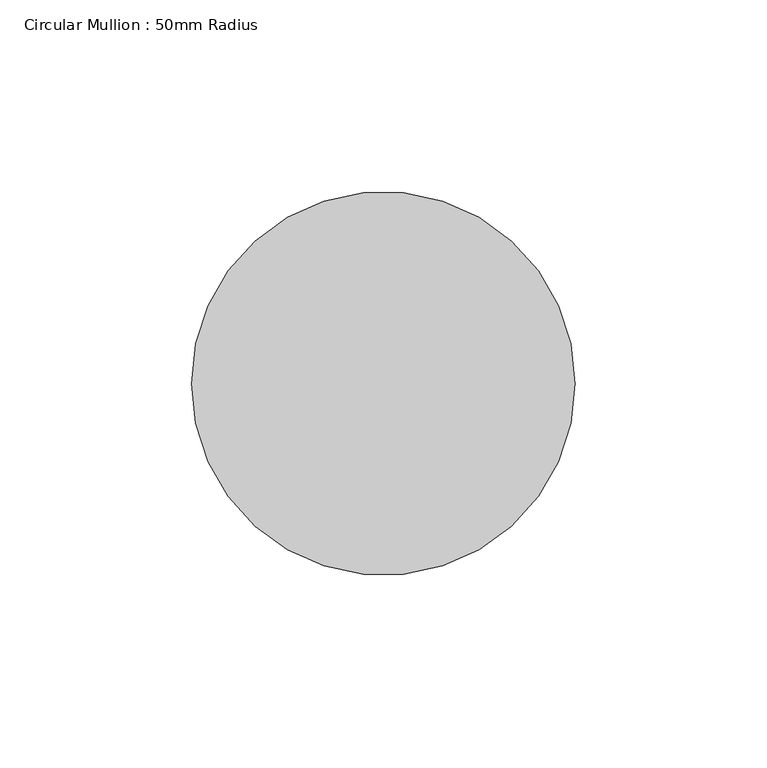
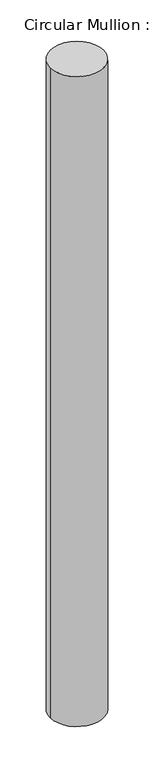
"""IFC4 building model written with IfcOpenShell, lengths in millimetres: member geometry, Circular Mullion : 50mm Radius."""

import ifcopenshell
import ifcopenshell.guid

model = None  # the IFC model being written
_history = None  # IfcOwnerHistory: only IFC2X3 demands one
_inside = {}  # id of a spatial element -> (the spatial element, [elements in it])
_under = {}  # id of a project, library or spatial element -> (it, [spatial elements below it])
_declared = {}  # id of a project -> (the project, [libraries it declares])
_typed = {}  # id of a type object -> (the type object, [elements of that type])
_made_of = {}  # id of a material, layer set ... -> (it, [elements and type objects made of it])


def new_model(schema):
    """Start an empty IFC model of exactly this schema.

    Asked for "IFC4X3", IfcOpenShell would pick the latest addendum, in which some entities
    have other attributes; the version numbers below select the first issue.
    IFC2X3 requires an IfcOwnerHistory on every rooted entity: one is made here for all.
    """
    global model, _history
    if schema == "IFC4X3":
        model = ifcopenshell.file(schema_version=(4, 3, 0, 0))
    else:
        model = ifcopenshell.file(schema=schema)
    _inside.clear()
    _under.clear()
    _declared.clear()
    _typed.clear()
    _made_of.clear()
    _history = None
    if model.schema == "IFC2X3":
        org = make("IfcOrganization", Name="unknown")
        user = make(
            "IfcPersonAndOrganization",
            ThePerson=make("IfcPerson", FamilyName="unknown"),
            TheOrganization=org,
        )
        app = make(
            "IfcApplication",
            ApplicationDeveloper=org,
            Version="unknown",
            ApplicationFullName="unknown",
            ApplicationIdentifier="unknown",
        )
        _history = make(
            "IfcOwnerHistory",
            OwningUser=user,
            OwningApplication=app,
            ChangeAction="ADDED",
            CreationDate=0,
        )
    return model


def make(cls, **values):
    """One entity of the class cls with the attributes given. An attribute that is None is left unset."""
    return model.create_entity(
        cls, **{name: value for name, value in values.items() if value is not None}
    )


def rooted(cls, **values):
    """An entity with a GlobalId (a new one), such as an element, a storey or a relation."""
    return make(cls, GlobalId=ifcopenshell.guid.new(), OwnerHistory=_history, **values)


def si_unit(unit_type, name, prefix=None):
    """IfcSIUnit, for example si_unit("LENGTHUNIT", "METRE", prefix="MILLI")."""
    return make("IfcSIUnit", UnitType=unit_type, Prefix=prefix, Name=name)


def assignment(units):
    """IfcUnitAssignment: the units of a project."""
    return None if units is None else make("IfcUnitAssignment", Units=units)


def point(xyz):
    """IfcCartesianPoint."""
    return None if xyz is None else make("IfcCartesianPoint", Coordinates=xyz)


def direction(xyz):
    """IfcDirection."""
    return None if xyz is None else make("IfcDirection", DirectionRatios=xyz)


def frame(location, z_axis=None, x_axis=None):
    """IfcAxis2Placement3D, a coordinate frame: its origin and axes. An axis left out is left unset."""
    return make(
        "IfcAxis2Placement3D",
        Location=point(location),
        Axis=direction(z_axis),
        RefDirection=direction(x_axis),
    )


def frame_2d(location, x_axis=None):
    """IfcAxis2Placement2D, a coordinate frame in the plane: its origin and x axis."""
    return make(
        "IfcAxis2Placement2D", Location=point(location), RefDirection=direction(x_axis)
    )


def origin():
    """The frame at (0, 0, 0) with its axes left unset."""
    return frame((0.0, 0.0, 0.0))


def origin_2d():
    """The frame at (0, 0) in the plane with its x axis left unset."""
    return frame_2d((0.0, 0.0))


def place(relative_to, where):
    """IfcLocalPlacement: puts the frame where relative to a parent placement (None: the world)."""
    return make(
        "IfcLocalPlacement", PlacementRelTo=relative_to, RelativePlacement=where
    )


def context(
    kind, dimensions, precision=None, world=None, true_north=None, identifier=None
):
    """IfcGeometricRepresentationContext, for example the 3D "Model" context."""
    return make(
        "IfcGeometricRepresentationContext",
        ContextIdentifier=identifier,
        ContextType=kind,
        CoordinateSpaceDimension=dimensions,
        Precision=precision,
        WorldCoordinateSystem=world,
        TrueNorth=true_north,
    )


def project(units=None, contexts=None):
    """IfcProject with its units and contexts."""
    return rooted(
        "IfcProject",
        Name="project",
        RepresentationContexts=contexts,
        UnitsInContext=assignment(units),
    )


def spatial(cls, under=None, at=None, **own):
    """A site, building, storey or space (cls), placed at a placement, below another one or the project."""
    s = rooted(cls, ObjectPlacement=at, **own)
    if under is not None:
        _under.setdefault(under.id(), (under, []))[1].append(s)
    return s


def circle_curve(where, radius):
    """IfcCircle in the frame where."""
    return make("IfcCircle", Position=where, Radius=radius)


def trimmed(basis, trim1, trim2, sense, master):
    """IfcTrimmedCurve: the piece of a basis curve between two trims."""
    return make(
        "IfcTrimmedCurve",
        BasisCurve=basis,
        Trim1=trim1,
        Trim2=trim2,
        SenseAgreement=sense,
        MasterRepresentation=master,
    )


def segment(curve, same_sense, transition):
    """IfcCompositeCurveSegment."""
    return make(
        "IfcCompositeCurveSegment",
        Transition=transition,
        SameSense=same_sense,
        ParentCurve=curve,
    )


def composite_curve(segments, self_intersect=None):
    """IfcCompositeCurve: segments joined end to end."""
    return make("IfcCompositeCurve", Segments=segments, SelfIntersect=self_intersect)


def outline(outer, holes=None, kind="AREA"):
    """IfcArbitraryClosedProfileDef: a profile drawn as a closed curve; with holes, ...WithVoids."""
    if holes is None:
        return make("IfcArbitraryClosedProfileDef", ProfileType=kind, OuterCurve=outer)
    return make(
        "IfcArbitraryProfileDefWithVoids",
        ProfileType=kind,
        OuterCurve=outer,
        InnerCurves=holes,
    )


def extrude(swept, where, along, depth):
    """IfcExtrudedAreaSolid: the profile swept, set in the frame where, extruded along a direction by depth."""
    return make(
        "IfcExtrudedAreaSolid",
        SweptArea=swept,
        Position=where,
        ExtrudedDirection=direction(along),
        Depth=depth,
    )


def shape(context_of_items, identifier, shape_type, items):
    """IfcShapeRepresentation: the items that make up one representation, for example the "Body"."""
    return make(
        "IfcShapeRepresentation",
        ContextOfItems=context_of_items,
        RepresentationIdentifier=identifier,
        RepresentationType=shape_type,
        Items=items,
    )


def source(mapping_origin, context_of_items, identifier, shape_type, items):
    """IfcRepresentationMap: a shape defined once, which mapped items show again and again."""
    return make(
        "IfcRepresentationMap",
        MappingOrigin=mapping_origin,
        MappedRepresentation=shape(context_of_items, identifier, shape_type, items),
    )


def transform(
    local_origin,
    x_axis=None,
    y_axis=None,
    z_axis=None,
    scale=None,
    scale2=None,
    scale3=None,
    uniform=True,
):
    """IfcCartesianTransformationOperator3D, or its non-uniform kind. x_axis, y_axis, z_axis: its Axis1, 2, 3."""
    if uniform:
        return make(
            "IfcCartesianTransformationOperator3D",
            Axis1=direction(x_axis),
            Axis2=direction(y_axis),
            LocalOrigin=point(local_origin),
            Scale=scale,
            Axis3=direction(z_axis),
        )
    return make(
        "IfcCartesianTransformationOperator3DnonUniform",
        Axis1=direction(x_axis),
        Axis2=direction(y_axis),
        LocalOrigin=point(local_origin),
        Scale=scale,
        Axis3=direction(z_axis),
        Scale2=scale2,
        Scale3=scale3,
    )


def mapped(mapping_source, mapping_target):
    """IfcMappedItem: shows the shape of a source again, moved by a transform."""
    return make(
        "IfcMappedItem", MappingSource=mapping_source, MappingTarget=mapping_target
    )


def made_of(thing, what):
    """Note that an element or type object is made of a material, layer set ...; save() writes the relation."""
    if what is not None:
        _made_of.setdefault(what.id(), (what, []))[1].append(thing)
    return thing


def element(
    cls,
    number,
    at=None,
    inside=None,
    cuts=None,
    type_object=None,
    material=None,
    context=None,
    identifier="Body",
    shape_type=None,
    held_by="IfcProductDefinitionShape",
    body=None,
    shapes=None,
    **own,
):
    """One element of the class cls, such as IfcWall. Its Tag is "e" and its number.

    at: its placement. inside: the storey or other place that contains it. cuts: it is an
    opening in that element (IfcRelVoidsElement). A single representation is given by context,
    identifier, shape_type and body (its items); several are given by shapes. held_by: the class
    of the entity that holds the representations. save() writes the other relations.
    """
    e = rooted(cls, Tag="e%d" % number, ObjectPlacement=at, **own)
    if body is not None:
        shapes = [shape(context, identifier, shape_type, body)]
    if shapes is not None:
        e.Representation = make(held_by, Representations=shapes)
    if inside is not None:
        _inside.setdefault(inside.id(), (inside, []))[1].append(e)
    if cuts is not None:
        rooted(
            "IfcRelVoidsElement", RelatingBuildingElement=cuts, RelatedOpeningElement=e
        )
    if type_object is not None:
        _typed.setdefault(type_object.id(), (type_object, []))[1].append(e)
    return made_of(e, material)


def aggregate(whole, parts):
    """IfcRelAggregates: a whole, such as a stair, and the parts it consists of."""
    return rooted("IfcRelAggregates", RelatingObject=whole, RelatedObjects=parts)


def save(model, path):
    """Write the relations noted so far, then the file.

    IfcRelAggregates (storeys below a building ...), IfcRelContainedInSpatialStructure (elements
    in a storey), IfcRelDefinesByType, IfcRelAssociatesMaterial and IfcRelDeclares: one each for
    every whole, place, type object, material and project.
    """
    for whole, parts in _under.values():
        aggregate(whole, parts)
    for where, things in _inside.values():
        rooted(
            "IfcRelContainedInSpatialStructure",
            RelatedElements=things,
            RelatingStructure=where,
        )
    for kind, things in _typed.values():
        rooted("IfcRelDefinesByType", RelatedObjects=things, RelatingType=kind)
    for what, things in _made_of.values():
        rooted("IfcRelAssociatesMaterial", RelatedObjects=things, RelatingMaterial=what)
    for by, libraries in _declared.values():
        rooted("IfcRelDeclares", RelatingContext=by, RelatedDefinitions=libraries)
    model.write(path)


def circular_mullion_50mm_radius_57aaed37(model_context):
    return source(origin(), model_context, "Body", "SweptSolid", [
        extrude(outline(composite_curve([segment(trimmed(circle_curve(origin_2d(), 50.0), [point((50.0, 0.0))], [point((-50.0, 0.0))], False, "CARTESIAN"), True, "CONTINUOUS"), segment(trimmed(circle_curve(origin_2d(), 50.0), [point((-50.0, 0.0))], [point((50.0, 0.0))], False, "CARTESIAN"), True, "CONTINUOUS")], self_intersect=False)), frame((0.0, 0.0, -1291.1086695), z_axis=(0.0, 0.0, 1.0), x_axis=(1.0, 0.0, 0.0)), (0.0, 0.0, 1.0), 1291.1086695),
    ])


if __name__ == "__main__":
    model = new_model("IFC4")
    model_context = context("Model", 3, world=origin())
    ifc_project = project(units=[si_unit("LENGTHUNIT", "METRE", prefix="MILLI")], contexts=[model_context])
    site = spatial("IfcSite", under=ifc_project)
    building = spatial("IfcBuilding", under=site)
    placement = place(None, origin())
    circular_mullion_50mm_radius_shape = circular_mullion_50mm_radius_57aaed37(model_context)
    element("IfcMember", 1, ObjectType="Circular Mullion : 50mm Radius", at=placement, inside=building, context=model_context, shape_type="MappedRepresentation", body=[
        mapped(circular_mullion_50mm_radius_shape, transform((0.0, 0.0, 0.0), x_axis=(1.0, 0.0, 0.0), y_axis=(0.0, 1.0, 0.0), z_axis=(0.0, 0.0, 1.0))),
    ])
    save(model, "model.ifc")

# Revit data of these elements
# Type "Circular Mullion : 50mm Radius"
#   built-in parameter 1007350 = 0.164042 (stored number, unit not read)
# Element 1 (IfcMember, "Circular Mullion : 50mm Radius")
#   Materials on its faces: "Aluminium"
# Materials
#   "Aluminium": class "Metal", colour RGB 247 247 247, transparency 0, Description = "Aluminium 6061", Cost = 0
